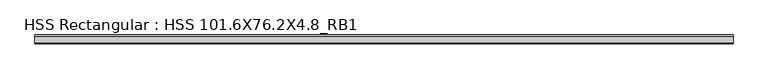
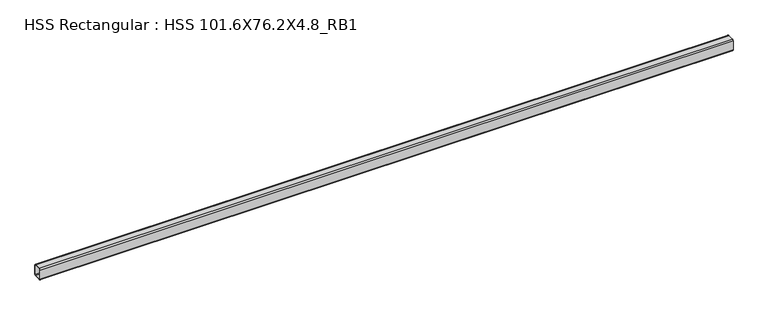
"""IFC4 building model written with IfcOpenShell, lengths in millimetres: beam geometry, HSS Rectangular : HSS 101.6X76.2X4.8_RB1."""

from ifc_helpers import new_model, si_unit, point, frame, frame_2d, origin, place, context, project, spatial, polyline, circle_curve, trimmed, segment, composite_curve, outline, extrude, source, transform, mapped, element, save


def hss_rectangular_hss_101_6x76_2x4_8_rb1_df13327d(model_context):
    return source(origin(), model_context, "Body", "SweptSolid", [
        extrude(outline(composite_curve([segment(polyline([(38.1, 41.275), (38.1, -41.275)]), True, "CONTINUOUS"), segment(trimmed(circle_curve(frame_2d((28.575, -41.275)), 9.525), [point((38.1, -41.275))], [point((28.575, -50.8))], False, "CARTESIAN"), True, "CONTINUOUS"), segment(polyline([(28.575, -50.8), (-28.575, -50.8)]), True, "CONTINUOUS"), segment(trimmed(circle_curve(frame_2d((-28.575, -41.275)), 9.525), [point((-28.575, -50.8))], [point((-38.1, -41.275))], False, "CARTESIAN"), True, "CONTINUOUS"), segment(polyline([(-38.1, -41.275), (-38.1, 41.275)]), True, "CONTINUOUS"), segment(trimmed(circle_curve(frame_2d((-28.575, 41.275)), 9.525), [point((-38.1, 41.275))], [point((-28.575, 50.8))], False, "CARTESIAN"), True, "CONTINUOUS"), segment(polyline([(-28.575, 50.8), (28.575, 50.8)]), True, "CONTINUOUS"), segment(trimmed(circle_curve(frame_2d((28.575, 41.275)), 9.525), [point((28.575, 50.8))], [point((38.1, 41.275))], False, "CARTESIAN"), True, "CONTINUOUS")], self_intersect=False), holes=[composite_curve([segment(trimmed(circle_curve(frame_2d((-28.575, 41.275)), 4.7625), [point((-28.575, 46.0375))], [point((-33.3375, 41.275))], True, "CARTESIAN"), True, "CONTINUOUS"), segment(polyline([(-33.3375, 41.275), (-33.3375, -41.275)]), True, "CONTINUOUS"), segment(trimmed(circle_curve(frame_2d((-28.575, -41.275)), 4.7625), [point((-33.3375, -41.275))], [point((-28.575, -46.0375))], True, "CARTESIAN"), True, "CONTINUOUS"), segment(polyline([(-28.575, -46.0375), (28.575, -46.0375)]), True, "CONTINUOUS"), segment(trimmed(circle_curve(frame_2d((28.575, -41.275)), 4.7625), [point((28.575, -46.0375))], [point((33.3375, -41.275))], True, "CARTESIAN"), True, "CONTINUOUS"), segment(polyline([(33.3375, -41.275), (33.3375, 41.275)]), True, "CONTINUOUS"), segment(trimmed(circle_curve(frame_2d((28.575, 41.275)), 4.7625), [point((33.3375, 41.275))], [point((28.575, 46.0375))], True, "CARTESIAN"), True, "CONTINUOUS"), segment(polyline([(28.575, 46.0375), (-28.575, 46.0375)]), True, "CONTINUOUS")], self_intersect=False)]), frame((-7451.011, 0.0, 0.0), z_axis=(1.0, 0.0, 0.0), x_axis=(0.0, 1.0, 0.0)), (0.0, 0.0, 1.0), 6014.511),
    ])


if __name__ == "__main__":
    model = new_model("IFC4")
    model_context = context("Model", 3, world=origin())
    ifc_project = project(units=[si_unit("LENGTHUNIT", "METRE", prefix="MILLI")], contexts=[model_context])
    site = spatial("IfcSite", under=ifc_project)
    building = spatial("IfcBuilding", under=site)
    placement = place(None, origin())
    hss_rectangular_hss_101_6x76_2x4_8_rb1_shape = hss_rectangular_hss_101_6x76_2x4_8_rb1_df13327d(model_context)
    element("IfcBeam", 1, ObjectType="HSS Rectangular : HSS 101.6X76.2X4.8_RB1", at=placement, inside=building, context=model_context, shape_type="MappedRepresentation", body=[
        mapped(hss_rectangular_hss_101_6x76_2x4_8_rb1_shape, transform((0.0, 0.0, 0.0), x_axis=(1.0, 0.0, 0.0), y_axis=(0.0, 1.0, 0.0), z_axis=(0.0, 0.0, 1.0))),
    ])
    save(model, "model.ifc")

# Revit data of these elements
# Type "HSS Rectangular : HSS 101.6X76.2X4.8_RB1"
#   Section Name Key = "HSS 4X3X3/16"
#   Assembly Code = "B10"
#   Width = 7.62 cm
#   Wall Nominal Thickness = 0.4763 cm
#   Wall Design Thickness = 0.442 cm
#   Torsional Moment of Inertia = 260.561 cm⁴
#   Torsional Modulus = 61.2876 cm³
#   Section Area = 14.4516 cm²
#   Plastic Modulus weak axis = 40.3122 cm³
#   Plastic Modulus strong axis = 49.1612 cm³
#   Perimeter = 0.881482 m²/m
#   Outer Fillet = 0.9525 cm
#   Nominal Weight = 12.1285 kgf/m
#   Moment of Inertia weak axis = 131.529 cm⁴
#   Moment of Inertia strong axis = 205.202 cm⁴
#   Inner Fillet = 0.4763 cm
#   Height = 10.16 cm
#   Elastic Modulus weak axis = 34.4128 cm³
#   Elastic Modulus strong axis = 40.476 cm³
#   Centroid Vertical = 5.08 cm
#   Centroid Horizontal = 3.81 cm
#   Length [instance default] = 1524 mm
#   Structural Material [instance default] = Steel ASTM A500, Grade B, Rectangular and Square
#   Principal Axes Angle = 0
# Element 1 (IfcBeam, "HSS Rectangular : HSS 101.6X76.2X4.8_RB1")
#   Structural Material = Steel ASTM A992
#   Materials on its faces: "Steel ASTM A992"
# Materials
#   "Steel ASTM A500, Grade B, Rectangular and Square": class "Metal", colour RGB 199 199 199, transparency 0, Description = "Carbon steel", Cost = 0
#   "Steel ASTM A992": class "Metal", colour RGB 199 199 199, transparency 0, Description = "Structural steel 50ksi", Cost = 0
